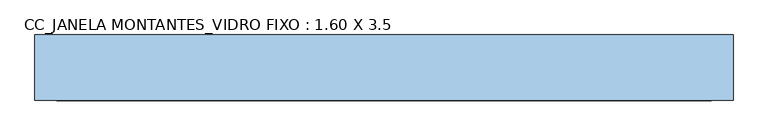
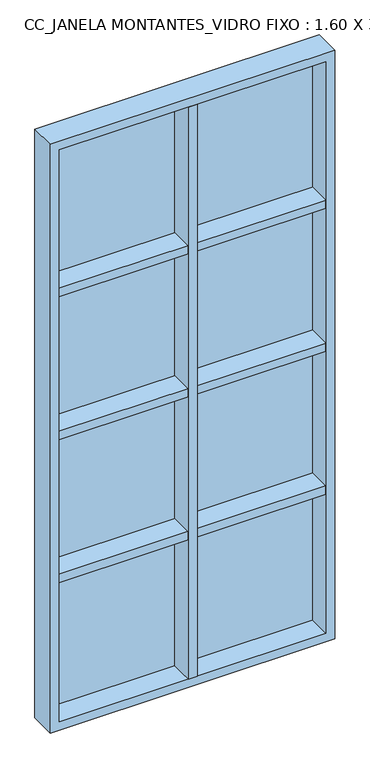
"""IFC4 building model written with IfcOpenShell, lengths in millimetres: window geometry, CC_JANELA MONTANTES_VIDRO FIXO : 1.60 X 3.5."""

from ifc_helpers import new_model, si_unit, frame, origin, place, context, project, spatial, polyline, outline, extrude, source, transform, mapped, element, save


def cc_janela_montantes_vidro_fixo_1_60_x_3_5_286e51ec(model_context):
    return source(origin(), model_context, "Body", "SweptSolid", [
        extrude(outline(polyline([(750.0, 97.5), (750.0, -47.5), (-750.0, -47.5), (-750.0, 97.5), (750.0, 97.5)])), frame((0.0, 0.0, 1875.0), z_axis=(0.0, 0.0, 1.0), x_axis=(1.0, 0.0, 0.0)), (0.0, 0.0, 1.0), 50.0),
        extrude(outline(polyline([(750.0, 97.5), (750.0, -47.5), (-750.0, -47.5), (-750.0, 97.5), (750.0, 97.5)])), frame((0.0, 0.0, 2725.0), z_axis=(0.0, 0.0, 1.0), x_axis=(1.0, 0.0, 0.0)), (0.0, 0.0, 1.0), 50.0),
        extrude(outline(polyline([(750.0, 97.5), (750.0, -47.5), (-750.0, -47.5), (-750.0, 97.5), (750.0, 97.5)])), frame((0.0, 0.0, 3575.0), z_axis=(0.0, 0.0, 1.0), x_axis=(1.0, 0.0, 0.0)), (0.0, 0.0, 1.0), 50.0),
        extrude(outline(polyline([(25.0, 100.0), (25.0, -50.0), (-25.0, -50.0), (-25.0, 100.0), (25.0, 100.0)])), frame((0.0, 0.0, 1050.0), z_axis=(0.0, 0.0, 1.0), x_axis=(1.0, 0.0, 0.0)), (0.0, 0.0, 1.0), 3400.0),
        extrude(outline(polyline([(4500.0, -800.0), (1000.0, -800.0), (1000.0, 800.0), (4500.0, 800.0), (4500.0, -800.0)]), holes=[polyline([(4450.0, -750.0), (4450.0, 750.0), (1050.0, 750.0), (1050.0, -750.0), (4450.0, -750.0)])]), frame((0.0, -50.0, 0.0), z_axis=(0.0, 1.0, 0.0), x_axis=(0.0, 0.0, 1.0)), (0.0, 0.0, 1.0), 150.0),
        extrude(outline(polyline([(750.0, 80.0), (-750.0, 80.0), (-750.0, 92.0), (750.0, 92.0), (750.0, 80.0)])), frame((0.0, 0.0, 1050.0), z_axis=(0.0, 0.0, 1.0), x_axis=(1.0, 0.0, 0.0)), (0.0, 0.0, 1.0), 3400.0),
    ])


if __name__ == "__main__":
    model = new_model("IFC4")
    model_context = context("Model", 3, world=origin())
    ifc_project = project(units=[si_unit("LENGTHUNIT", "METRE", prefix="MILLI")], contexts=[model_context])
    site = spatial("IfcSite", under=ifc_project)
    building = spatial("IfcBuilding", under=site)
    placement = place(None, origin())
    cc_janela_montantes_vidro_fixo_1_60_x_3_5_shape = cc_janela_montantes_vidro_fixo_1_60_x_3_5_286e51ec(model_context)
    element("IfcWindow", 1, ObjectType="CC_JANELA MONTANTES_VIDRO FIXO : 1.60 X 3.5", at=placement, inside=building, context=model_context, shape_type="MappedRepresentation", body=[
        mapped(cc_janela_montantes_vidro_fixo_1_60_x_3_5_shape, transform((0.0, 0.0, 0.0), x_axis=(1.0, 0.0, 0.0), y_axis=(0.0, 1.0, 0.0), z_axis=(0.0, 0.0, 1.0))),
    ])
    save(model, "model.ifc")

# Revit data of these elements
# Type "CC_JANELA MONTANTES_VIDRO FIXO : 1.60 X 3.5"
#   Type Mark = "J9"
#   Analytic Construction = "<Nenhum>"
#   Largura janela = 1.50 m
#   Espaçamento montantes verticais [instance default] = 0.75 m
#   Espaçamento montantes horizontais [instance default] = 0.85 m
#   Altura janela = 3.40 m
#   Height = 3.50 m
#   Altura-padrão do peitoril = 1.00 m
#   Width = 1.60 m
#   N verticais [instance default] = 2
#   N horizontais [instance default] = 3
#   N de montantes verticais [instance default] = 1
#   N de montantes horizontais [instance default] = 3
#   Montate vertical vários [instance default] = no
#   Montante vertical único [instance default] = yes
#   Montante horizontal único [instance default] = no
#   Montante horizontal vários [instance default] = yes
#   Tipo de vidro = .VIDRO
#   Material da esquadria = .ALUMÍNIO COM PINTURA ELETROSTÁTICA BRANCA
#   Wall Closure = (empty or 0)
# Element 1 (IfcWindow, "CC_JANELA MONTANTES_VIDRO FIXO : 1.60 X 3.5")
#   Materials on its faces: ".ALUMÍNIO COM PINTURA ELETROSTÁTICA BRANCA", ".VIDRO"
# Materials
#   ".VIDRO": class "Genérico", colour RGB 198 236 255, transparency 0.95, Cost = 0
#   ".ALUMÍNIO COM PINTURA ELETROSTÁTICA BRANCA": class "CC_METAIS", colour RGB 241 241 241, transparency 0, Cost = 0
